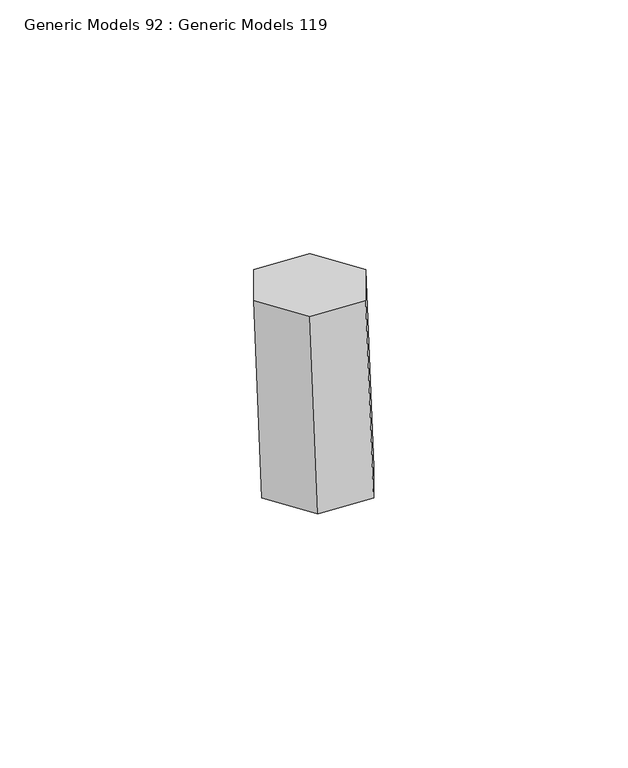
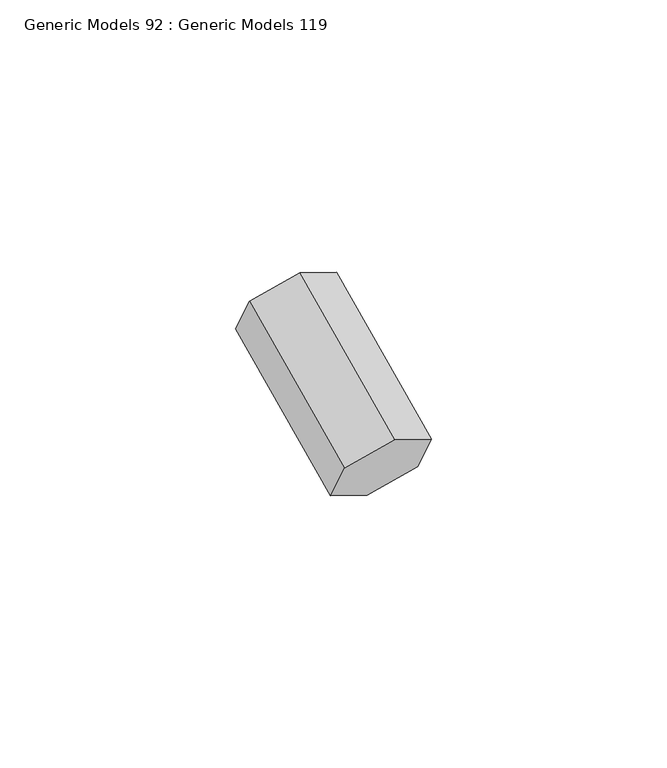
"""IFC4 building model written with IfcOpenShell, lengths in millimetres: proxy geometry, Generic Models 92 : Generic Models 119."""

from ifc_helpers import new_model, si_unit, origin, place, context, project, spatial, faceted_brep, source, transform, mapped, element, save


def generic_models_92_generic_models_119_97e9f889(model_context):
    return source(origin(), model_context, "Body", "Brep", [
        faceted_brep([(31992.9980552, 35130.542011, 271586.7128013), (31992.9980552, 35136.6990932, 271575.605131), (32003.9965778, 35139.7776342, 271570.0512959), (32014.9951004, 35136.6990932, 271575.605131), (32014.9951004, 35130.542011, 271586.7128013), (32003.9965778, 35127.4634699, 271592.2666364), (31991.446556, 35169.418857, 271608.2625889), (32002.4450787, 35166.3403159, 271613.816424), (32013.4436013, 35169.418857, 271608.2625889), (32013.4436013, 35175.5759391, 271597.1549186), (32002.4450787, 35178.6544802, 271591.6010835), (31991.446556, 35175.5759391, 271597.1549186)], [[[0, 1, 2, 3, 4, 5]], [[6, 7, 8, 9, 10, 11]], [[6, 11, 1, 0]], [[11, 10, 2, 1]], [[10, 9, 3, 2]], [[9, 8, 4, 3]], [[8, 7, 5, 4]], [[7, 6, 0, 5]]]),
    ])


if __name__ == "__main__":
    model = new_model("IFC4")
    model_context = context("Model", 3, world=origin())
    ifc_project = project(units=[si_unit("LENGTHUNIT", "METRE", prefix="MILLI")], contexts=[model_context])
    site = spatial("IfcSite", under=ifc_project)
    building = spatial("IfcBuilding", under=site)
    placement = place(None, origin())
    generic_models_92_generic_models_119_shape = generic_models_92_generic_models_119_97e9f889(model_context)
    element("IfcBuildingElementProxy", 1, Name="Generic Models 92 : Generic Models 119", ObjectType="Generic Models 92 : Generic Models 119", at=placement, inside=building, context=model_context, shape_type="MappedRepresentation", body=[
        mapped(generic_models_92_generic_models_119_shape, transform((0.0, 0.0, 0.0), x_axis=(1.0, 0.0, 0.0), y_axis=(0.0, 1.0, 0.0), z_axis=(0.0, 0.0, 1.0))),
    ])
    save(model, "model.ifc")
